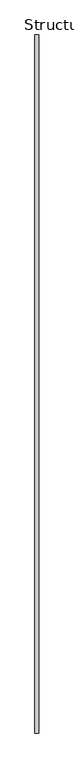
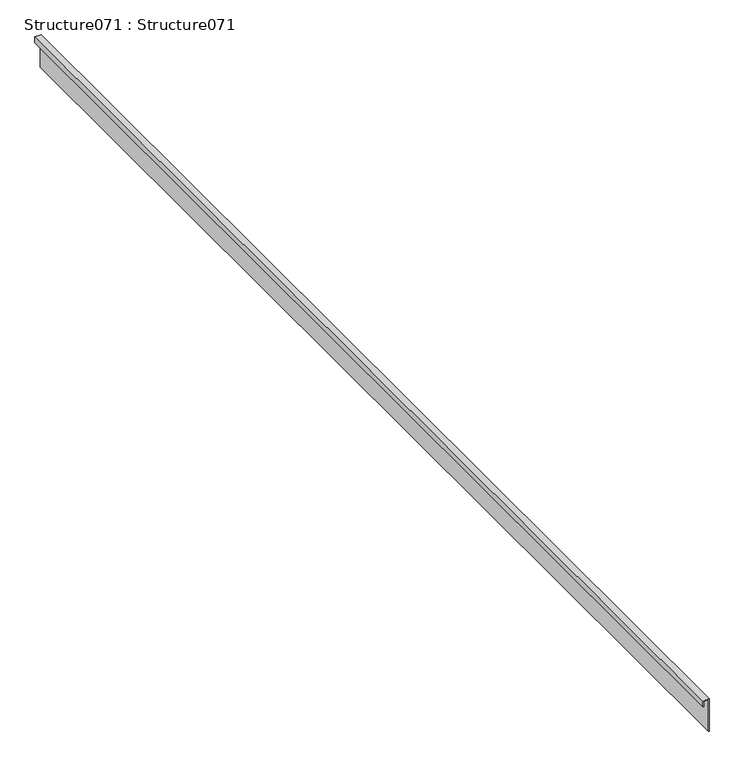
"""IFC4 building model written with IfcOpenShell, lengths in millimetres: proxy geometry, Structure071 : Structure071."""

import ifcopenshell
import ifcopenshell.guid

model = None  # the IFC model being written
_history = None  # IfcOwnerHistory: only IFC2X3 demands one
_inside = {}  # id of a spatial element -> (the spatial element, [elements in it])
_under = {}  # id of a project, library or spatial element -> (it, [spatial elements below it])
_declared = {}  # id of a project -> (the project, [libraries it declares])
_typed = {}  # id of a type object -> (the type object, [elements of that type])
_made_of = {}  # id of a material, layer set ... -> (it, [elements and type objects made of it])


def new_model(schema):
    """Start an empty IFC model of exactly this schema.

    Asked for "IFC4X3", IfcOpenShell would pick the latest addendum, in which some entities
    have other attributes; the version numbers below select the first issue.
    IFC2X3 requires an IfcOwnerHistory on every rooted entity: one is made here for all.
    """
    global model, _history
    if schema == "IFC4X3":
        model = ifcopenshell.file(schema_version=(4, 3, 0, 0))
    else:
        model = ifcopenshell.file(schema=schema)
    _inside.clear()
    _under.clear()
    _declared.clear()
    _typed.clear()
    _made_of.clear()
    _history = None
    if model.schema == "IFC2X3":
        org = make("IfcOrganization", Name="unknown")
        user = make(
            "IfcPersonAndOrganization",
            ThePerson=make("IfcPerson", FamilyName="unknown"),
            TheOrganization=org,
        )
        app = make(
            "IfcApplication",
            ApplicationDeveloper=org,
            Version="unknown",
            ApplicationFullName="unknown",
            ApplicationIdentifier="unknown",
        )
        _history = make(
            "IfcOwnerHistory",
            OwningUser=user,
            OwningApplication=app,
            ChangeAction="ADDED",
            CreationDate=0,
        )
    return model


def make(cls, **values):
    """One entity of the class cls with the attributes given. An attribute that is None is left unset."""
    return model.create_entity(
        cls, **{name: value for name, value in values.items() if value is not None}
    )


def rooted(cls, **values):
    """An entity with a GlobalId (a new one), such as an element, a storey or a relation."""
    return make(cls, GlobalId=ifcopenshell.guid.new(), OwnerHistory=_history, **values)


def si_unit(unit_type, name, prefix=None):
    """IfcSIUnit, for example si_unit("LENGTHUNIT", "METRE", prefix="MILLI")."""
    return make("IfcSIUnit", UnitType=unit_type, Prefix=prefix, Name=name)


def assignment(units):
    """IfcUnitAssignment: the units of a project."""
    return None if units is None else make("IfcUnitAssignment", Units=units)


def point(xyz):
    """IfcCartesianPoint."""
    return None if xyz is None else make("IfcCartesianPoint", Coordinates=xyz)


def direction(xyz):
    """IfcDirection."""
    return None if xyz is None else make("IfcDirection", DirectionRatios=xyz)


def frame(location, z_axis=None, x_axis=None):
    """IfcAxis2Placement3D, a coordinate frame: its origin and axes. An axis left out is left unset."""
    return make(
        "IfcAxis2Placement3D",
        Location=point(location),
        Axis=direction(z_axis),
        RefDirection=direction(x_axis),
    )


def origin():
    """The frame at (0, 0, 0) with its axes left unset."""
    return frame((0.0, 0.0, 0.0))


def place(relative_to, where):
    """IfcLocalPlacement: puts the frame where relative to a parent placement (None: the world)."""
    return make(
        "IfcLocalPlacement", PlacementRelTo=relative_to, RelativePlacement=where
    )


def context(
    kind, dimensions, precision=None, world=None, true_north=None, identifier=None
):
    """IfcGeometricRepresentationContext, for example the 3D "Model" context."""
    return make(
        "IfcGeometricRepresentationContext",
        ContextIdentifier=identifier,
        ContextType=kind,
        CoordinateSpaceDimension=dimensions,
        Precision=precision,
        WorldCoordinateSystem=world,
        TrueNorth=true_north,
    )


def project(units=None, contexts=None):
    """IfcProject with its units and contexts."""
    return rooted(
        "IfcProject",
        Name="project",
        RepresentationContexts=contexts,
        UnitsInContext=assignment(units),
    )


def spatial(cls, under=None, at=None, **own):
    """A site, building, storey or space (cls), placed at a placement, below another one or the project."""
    s = rooted(cls, ObjectPlacement=at, **own)
    if under is not None:
        _under.setdefault(under.id(), (under, []))[1].append(s)
    return s


def polyline(points):
    """IfcPolyline through the points."""
    return make("IfcPolyline", Points=[point(p) for p in points])


def outline(outer, holes=None, kind="AREA"):
    """IfcArbitraryClosedProfileDef: a profile drawn as a closed curve; with holes, ...WithVoids."""
    if holes is None:
        return make("IfcArbitraryClosedProfileDef", ProfileType=kind, OuterCurve=outer)
    return make(
        "IfcArbitraryProfileDefWithVoids",
        ProfileType=kind,
        OuterCurve=outer,
        InnerCurves=holes,
    )


def extrude(swept, where, along, depth):
    """IfcExtrudedAreaSolid: the profile swept, set in the frame where, extruded along a direction by depth."""
    return make(
        "IfcExtrudedAreaSolid",
        SweptArea=swept,
        Position=where,
        ExtrudedDirection=direction(along),
        Depth=depth,
    )


def shape(context_of_items, identifier, shape_type, items):
    """IfcShapeRepresentation: the items that make up one representation, for example the "Body"."""
    return make(
        "IfcShapeRepresentation",
        ContextOfItems=context_of_items,
        RepresentationIdentifier=identifier,
        RepresentationType=shape_type,
        Items=items,
    )


def source(mapping_origin, context_of_items, identifier, shape_type, items):
    """IfcRepresentationMap: a shape defined once, which mapped items show again and again."""
    return make(
        "IfcRepresentationMap",
        MappingOrigin=mapping_origin,
        MappedRepresentation=shape(context_of_items, identifier, shape_type, items),
    )


def transform(
    local_origin,
    x_axis=None,
    y_axis=None,
    z_axis=None,
    scale=None,
    scale2=None,
    scale3=None,
    uniform=True,
):
    """IfcCartesianTransformationOperator3D, or its non-uniform kind. x_axis, y_axis, z_axis: its Axis1, 2, 3."""
    if uniform:
        return make(
            "IfcCartesianTransformationOperator3D",
            Axis1=direction(x_axis),
            Axis2=direction(y_axis),
            LocalOrigin=point(local_origin),
            Scale=scale,
            Axis3=direction(z_axis),
        )
    return make(
        "IfcCartesianTransformationOperator3DnonUniform",
        Axis1=direction(x_axis),
        Axis2=direction(y_axis),
        LocalOrigin=point(local_origin),
        Scale=scale,
        Axis3=direction(z_axis),
        Scale2=scale2,
        Scale3=scale3,
    )


def mapped(mapping_source, mapping_target):
    """IfcMappedItem: shows the shape of a source again, moved by a transform."""
    return make(
        "IfcMappedItem", MappingSource=mapping_source, MappingTarget=mapping_target
    )


def made_of(thing, what):
    """Note that an element or type object is made of a material, layer set ...; save() writes the relation."""
    if what is not None:
        _made_of.setdefault(what.id(), (what, []))[1].append(thing)
    return thing


def element(
    cls,
    number,
    at=None,
    inside=None,
    cuts=None,
    type_object=None,
    material=None,
    context=None,
    identifier="Body",
    shape_type=None,
    held_by="IfcProductDefinitionShape",
    body=None,
    shapes=None,
    **own,
):
    """One element of the class cls, such as IfcWall. Its Tag is "e" and its number.

    at: its placement. inside: the storey or other place that contains it. cuts: it is an
    opening in that element (IfcRelVoidsElement). A single representation is given by context,
    identifier, shape_type and body (its items); several are given by shapes. held_by: the class
    of the entity that holds the representations. save() writes the other relations.
    """
    e = rooted(cls, Tag="e%d" % number, ObjectPlacement=at, **own)
    if body is not None:
        shapes = [shape(context, identifier, shape_type, body)]
    if shapes is not None:
        e.Representation = make(held_by, Representations=shapes)
    if inside is not None:
        _inside.setdefault(inside.id(), (inside, []))[1].append(e)
    if cuts is not None:
        rooted(
            "IfcRelVoidsElement", RelatingBuildingElement=cuts, RelatedOpeningElement=e
        )
    if type_object is not None:
        _typed.setdefault(type_object.id(), (type_object, []))[1].append(e)
    return made_of(e, material)


def aggregate(whole, parts):
    """IfcRelAggregates: a whole, such as a stair, and the parts it consists of."""
    return rooted("IfcRelAggregates", RelatingObject=whole, RelatedObjects=parts)


def save(model, path):
    """Write the relations noted so far, then the file.

    IfcRelAggregates (storeys below a building ...), IfcRelContainedInSpatialStructure (elements
    in a storey), IfcRelDefinesByType, IfcRelAssociatesMaterial and IfcRelDeclares: one each for
    every whole, place, type object, material and project.
    """
    for whole, parts in _under.values():
        aggregate(whole, parts)
    for where, things in _inside.values():
        rooted(
            "IfcRelContainedInSpatialStructure",
            RelatedElements=things,
            RelatingStructure=where,
        )
    for kind, things in _typed.values():
        rooted("IfcRelDefinesByType", RelatedObjects=things, RelatingType=kind)
    for what, things in _made_of.values():
        rooted("IfcRelAssociatesMaterial", RelatedObjects=things, RelatingMaterial=what)
    for by, libraries in _declared.values():
        rooted("IfcRelDeclares", RelatingContext=by, RelatedDefinitions=libraries)
    model.write(path)


def structure071_structure071_913a2800(model_context):
    return source(origin(), model_context, "Body", "SweptSolid", [
        extrude(outline(polyline([(42624.3685095, 5847.416096), (42624.3685095, 5848.606721), (42634.0, 5848.606721), (42634.0, 5856.8662109), (42576.61192, 5856.8662109), (42576.61192, 5858.0568359), (42635.190625, 5858.0568359), (42635.190625, 5847.416096), (42624.3685095, 5847.416096)])), frame((0.0, -1052.8906574, 0.0), z_axis=(0.0, 1.0, 0.0), x_axis=(0.0, 0.0, 1.0)), (0.0, 0.0, 1.0), 1999.85),
    ])


if __name__ == "__main__":
    model = new_model("IFC4")
    model_context = context("Model", 3, world=origin())
    ifc_project = project(units=[si_unit("LENGTHUNIT", "METRE", prefix="MILLI")], contexts=[model_context])
    site = spatial("IfcSite", under=ifc_project)
    building = spatial("IfcBuilding", under=site)
    placement = place(None, origin())
    structure071_structure071_shape = structure071_structure071_913a2800(model_context)
    element("IfcBuildingElementProxy", 1, Name="Structure071 : Structure071", ObjectType="Structure071 : Structure071", at=placement, inside=building, context=model_context, shape_type="MappedRepresentation", body=[
        mapped(structure071_structure071_shape, transform((0.0, 0.0, 0.0), x_axis=(1.0, 0.0, 0.0), y_axis=(0.0, 1.0, 0.0), z_axis=(0.0, 0.0, 1.0))),
    ])
    save(model, "model.ifc")

# Revit data of these elements
# Type "Structure071 : Structure071"
#   NameOverride = "Structure071"
# Element 1 (IfcBuildingElementProxy, "Structure071 : Structure071")
#   Materials on its faces: "STANDING SEAM METAL ROOF FOLLOW MANU. RECOMMENDED EDGE/TRANSITION DETAILS"
# Materials
#   "STANDING SEAM METAL ROOF FOLLOW MANU. RECOMMENDED EDGE/TRANSITION DETAILS": class "Unassigned", colour RGB 128 128 128, transparency 0, Cost = 0
